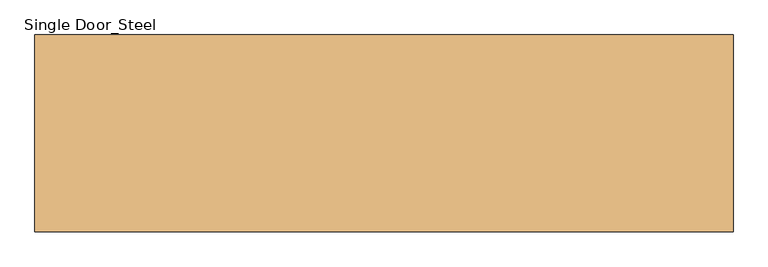
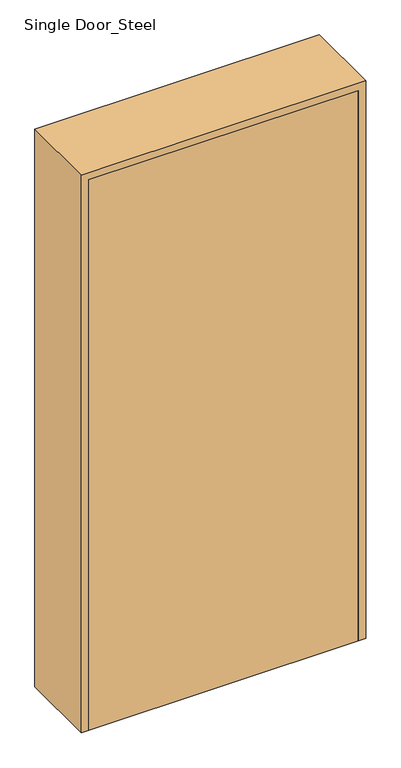
"""IFC4 building model written with IfcOpenShell, lengths in millimetres: door geometry, Single Door_Steel : H_DR_AR_B12_Single Door_Steel_W1100xH2280_SD1."""

from ifc_helpers import new_model, si_unit, origin, origin_with_axes, place, context, project, spatial, polyline, outline, extrude, faceted_brep, source, transform, mapped, element, save


def single_door_steel_0719061a(model_context):
    return source(origin(), model_context, "Body", "SolidModel", [
        extrude(outline(polyline([(520.0, -155.0), (-520.0, -155.0), (-520.0, -120.0), (520.0, -120.0), (520.0, -155.0)])), origin_with_axes(), (0.0, 0.0, 1.0), 2250.0),
        faceted_brep([(520.0, -155.0, 0.0), (520.0, -120.0, 0.0), (500.0, -120.0, 0.0), (500.0, 120.0, 0.0), (520.0, 120.0, 0.0), (520.0, 155.0, 0.0), (550.0, 155.0, 0.0), (550.0, -155.0, 0.0), (550.0, -155.0, 2280.0), (-550.0, -155.0, 2280.0), (-550.0, -155.0, 0.0), (-520.0, -155.0, 0.0), (-520.0, -155.0, 2250.0), (520.0, -155.0, 2250.0), (550.0, 155.0, 2280.0), (520.0, 155.0, 2250.0), (-520.0, 155.0, 2250.0), (-520.0, 155.0, 0.0), (-550.0, 155.0, 0.0), (-550.0, 155.0, 2280.0), (520.0, 120.0, 2250.0), (500.0, 120.0, 2230.0), (-500.0, 120.0, 2230.0), (-500.0, 120.0, 0.0), (-520.0, 120.0, 0.0), (-520.0, 120.0, 2250.0), (500.0, -120.0, 2230.0), (520.0, -120.0, 2250.0), (-520.0, -120.0, 2250.0), (-520.0, -120.0, 0.0), (-500.0, -120.0, 0.0), (-500.0, -120.0, 2230.0)], [[[0, 1, 2, 3, 4, 5, 6, 7]], [[7, 8, 9, 10, 11, 12, 13, 0]], [[6, 14, 8, 7]], [[5, 15, 16, 17, 18, 19, 14, 6]], [[4, 20, 15, 5]], [[3, 21, 22, 23, 24, 25, 20, 4]], [[2, 26, 21, 3]], [[1, 27, 28, 29, 30, 31, 26, 2]], [[0, 13, 27, 1]], [[12, 11, 29, 28]], [[11, 10, 18, 17, 24, 23, 30, 29]], [[19, 18, 10, 9]], [[25, 24, 17, 16]], [[31, 30, 23, 22]], [[14, 19, 9, 8]], [[20, 25, 16, 15]], [[26, 31, 22, 21]], [[13, 12, 28, 27]]]),
    ])


if __name__ == "__main__":
    model = new_model("IFC4")
    model_context = context("Model", 3, world=origin())
    ifc_project = project(units=[si_unit("LENGTHUNIT", "METRE", prefix="MILLI")], contexts=[model_context])
    site = spatial("IfcSite", under=ifc_project)
    building = spatial("IfcBuilding", under=site)
    placement = place(None, origin())
    single_door_steel_shape = single_door_steel_0719061a(model_context)
    element("IfcDoor", 1, ObjectType="Single Door_Steel : H_DR_AR_B12_Single Door_Steel_W1100xH2280_SD1", at=placement, inside=building, context=model_context, shape_type="MappedRepresentation", body=[
        mapped(single_door_steel_shape, transform((0.0, 0.0, 0.0), x_axis=(1.0, 0.0, 0.0), y_axis=(0.0, 1.0, 0.0), z_axis=(0.0, 0.0, 1.0))),
    ])
    save(model, "model.ifc")

# Revit data of these elements
# Type "Single Door_Steel : H_DR_AR_B12_Single Door_Steel_W1100xH2280_SD1"
#   Type Mark = "430"
#   Analytic Construction = "<None>"
#   프레임 투영 외부. = 25 mm
#   프레임 투영 내부. = 25 mm
#   프레임 폭 = 75 mm
#   Height = 2280 mm
#   Width = 1100 mm
#   Define Thermal Properties by = 1
#   문 패널 = none
#   문 프레임 = none
#   Function = (empty or 0)
#   Wall Closure = (empty or 0)
